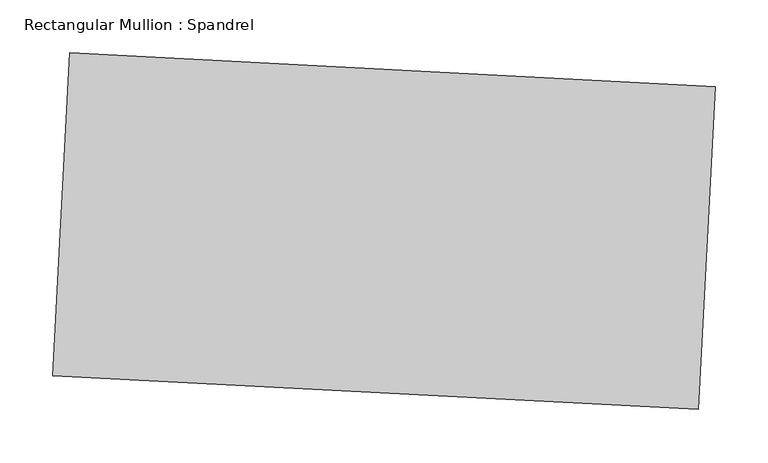
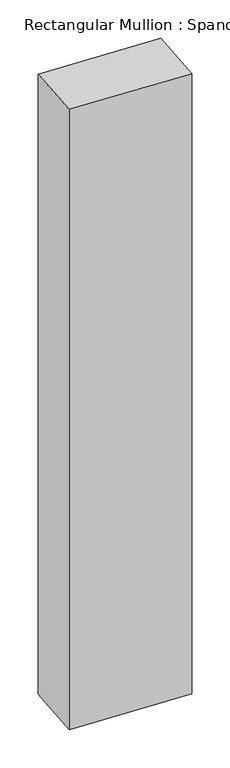
"""IFC4 building model written with IfcOpenShell, lengths in millimetres: member geometry, Rectangular Mullion : Spandrel."""

from ifc_helpers import new_model, si_unit, frame, origin, place, context, project, spatial, polyline, outline, extrude, source, transform, mapped, element, save


def rectangular_mullion_spandrel_e4d64f46(model_context):
    return source(origin(), model_context, "Body", "SweptSolid", [
        extrude(outline(polyline([(7.5582819, 136.2391416), (-8.3937175, -168.1431406), (-617.1582819, -136.2391416), (-601.2062825, 168.1431406), (7.5582819, 136.2391416)])), frame((0.0, 0.0, -3352.8), z_axis=(0.0, 0.0, 1.0), x_axis=(1.0, 0.0, 0.0)), (0.0, 0.0, 1.0), 3352.8),
    ])


if __name__ == "__main__":
    model = new_model("IFC4")
    model_context = context("Model", 3, world=origin())
    ifc_project = project(units=[si_unit("LENGTHUNIT", "METRE", prefix="MILLI")], contexts=[model_context])
    site = spatial("IfcSite", under=ifc_project)
    building = spatial("IfcBuilding", under=site)
    placement = place(None, origin())
    rectangular_mullion_spandrel_shape = rectangular_mullion_spandrel_e4d64f46(model_context)
    element("IfcMember", 1, ObjectType="Rectangular Mullion : Spandrel", at=placement, inside=building, context=model_context, shape_type="MappedRepresentation", body=[
        mapped(rectangular_mullion_spandrel_shape, transform((0.0, 0.0, 0.0), x_axis=(1.0, 0.0, 0.0), y_axis=(0.0, 1.0, 0.0), z_axis=(0.0, 0.0, 1.0))),
    ])
    save(model, "model.ifc")

# Revit data of these elements
# Type "Rectangular Mullion : Spandrel"
#   built-in parameter 1007304 = 1 (stored number, unit not read)
#   built-in parameter 1007301 = 1 (stored number, unit not read)
#   built-in parameter 1007300 = 1 (stored number, unit not read)
# Element 1 (IfcMember, "Rectangular Mullion : Spandrel")
#   Materials on its faces: "Aluminum"
# Materials
#   "Aluminum": class "Metal", colour RGB 247 247 247, transparency 0, Description = "Aluminum 6061", Cost = 0
